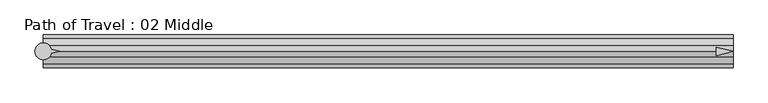
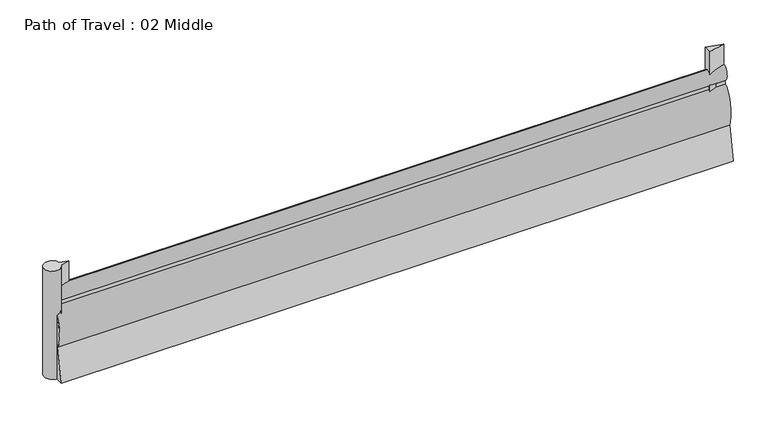
"""IFC4 building model written with IfcOpenShell, lengths in millimetres: proxy geometry, Path of Travel : 02 Middle."""

from ifc_helpers import new_model, si_unit, point, frame, frame_2d, origin, origin_with_axes, place, context, project, spatial, polyline, circle_curve, ellipse_curve, trimmed, segment, composite_curve, outline, extrude, source, transform, mapped, element, save
from ifc_brep_helpers import plane_surface, extruded_surface, advanced_brep


def path_of_travel_02_middle_b8d1a797(model_context):
    return source(origin(), model_context, "Body", "SolidModel", [
        advanced_brep(
        [(227.5554837, 0.0, 1727.2), (227.5554837, 42.9018657, 1436.6534209), (227.5554837, 42.9018657, 1363.4763406), (227.5554837, 184.1186263, 643.4144547), (227.5554837, 297.5699544, 0.0), (227.5554837, 145.6574193, 0.0), (227.5554837, 0.0, 584.2), (227.5554837, -145.6574193, 0.0), (227.5554837, -297.5699544, 0.0), (227.5554837, -184.1186263, 643.4144547), (227.5554837, -42.9018657, 1363.4763406), (227.5554837, -42.9018657, 1436.6534209), (12742.5650369, 0.0, 1727.2), (12742.5650369, -42.9018657, 1436.6534209), (12742.5650369, -42.9018657, 1363.4763406), (12742.5650369, -184.1186263, 643.4144547), (12742.5650369, -297.5699544, 0.0), (12742.5650369, -145.6574193, 0.0), (12742.5650369, 0.0, 584.2), (12742.5650369, 145.6574193, 0.0), (12742.5650369, 297.5699544, 0.0), (12742.5650369, 184.1186263, 643.4144547), (12742.5650369, 42.9018657, 1363.4763406), (12742.5650369, 42.9018657, 1436.6534209)],
        [
            (0, 1, ellipse_curve(frame((227.5554837, 0.0, 1574.8), z_axis=(-1.0, 0.0, 0.0), x_axis=(0.0, 0.0, 1.0)), 152.4, 101.6)),
            (1, 2),
            (2, 3, ellipse_curve(frame((227.5554837, 0.0, 914.4), z_axis=(-1.0, 0.0, 0.0), x_axis=(0.0, 0.0, -1.0)), 457.2, 228.6)),
            (3, 4),
            (4, 5),
            (5, 6),
            (6, 7),
            (7, 8),
            (8, 9),
            (9, 10, ellipse_curve(frame((227.5554837, 0.0, 914.4), z_axis=(-1.0, 0.0, 0.0), x_axis=(0.0, 0.0, -1.0)), 457.2, 228.6)),
            (10, 11),
            (11, 0, ellipse_curve(frame((227.5554837, 0.0, 1574.8), z_axis=(-1.0, 0.0, 0.0), x_axis=(0.0, 0.0, 1.0)), 152.4, 101.6)),
            (12, 13, ellipse_curve(frame((12742.5650369, 0.0, 1574.8), z_axis=(1.0, 0.0, 0.0), x_axis=(0.0, 0.0, 1.0)), 152.4, 101.6)),
            (13, 14),
            (14, 15, ellipse_curve(frame((12742.5650369, 0.0, 914.4), z_axis=(1.0, 0.0, 0.0), x_axis=(0.0, 0.0, -1.0)), 457.2, 228.6)),
            (15, 16),
            (16, 17),
            (17, 18),
            (18, 19),
            (19, 20),
            (20, 21),
            (21, 22, ellipse_curve(frame((12742.5650369, 0.0, 914.4), z_axis=(1.0, 0.0, 0.0), x_axis=(0.0, 0.0, -1.0)), 457.2, 228.6)),
            (22, 23),
            (23, 12, ellipse_curve(frame((12742.5650369, 0.0, 1574.8), z_axis=(1.0, 0.0, 0.0), x_axis=(0.0, 0.0, 1.0)), 152.4, 101.6)),
            (0, 12),
            (23, 1),
            (22, 2),
            (21, 3),
            (20, 4),
            (19, 5),
            (18, 6),
            (17, 7),
            (16, 8),
            (15, 9),
            (14, 10),
            (13, 11),
        ],
        [
            plane_surface(frame((227.5554837, 0.0, 0.0), z_axis=(-1.0, 0.0, 0.0), x_axis=(0.0, 0.0, 1.0))),
            plane_surface(frame((12742.5650369, 0.0, 0.0), z_axis=(1.0, 0.0, 0.0), x_axis=(0.0, 0.0, 1.0))),
            extruded_surface(trimmed(ellipse_curve(frame((12742.5650369, 0.0, 1574.8), z_axis=(-1.0, 0.0, 0.0), x_axis=(0.0, 0.0, 1.0)), 152.4, 101.6), [point((12742.5650369, 0.0, 1727.2))], [point((12742.5650369, 42.9018657, 1436.6534209))], True, "CARTESIAN"), (-12515.0095532, 0.0, 0.0), 12515.0095532),
            plane_surface(frame((227.5554837, 42.9018657, 1436.6534209), z_axis=(0.0, 1.0, 0.0), x_axis=(1.0, 0.0, 0.0))),
            extruded_surface(trimmed(ellipse_curve(frame((12742.5650369, 0.0, 914.4), z_axis=(-1.0, 0.0, 0.0), x_axis=(0.0, 0.0, -1.0)), 457.2, 228.6), [point((12742.5650369, 42.9018657, 1363.4763406))], [point((12742.5650369, 184.1186263, 643.4144547))], True, "CARTESIAN"), (-12515.0095532, 0.0, 0.0), 12515.0095532),
            plane_surface(frame((227.5554837, 184.1186263, 643.4144547), z_axis=(0.0, 0.9848077530122078, 0.1736481776669322), x_axis=(1.0, 0.0, 0.0))),
            plane_surface(frame((227.5554837, 297.5699544, 0.0), z_axis=(0.0, 0.0, -1.0), x_axis=(1.0, 0.0, 0.0))),
            plane_surface(frame((227.5554837, 145.6574193, 0.0), z_axis=(0.0, -0.9702957262760199, -0.2419218955995739), x_axis=(1.0, 0.0, 0.0))),
            plane_surface(frame((227.5554837, 0.0, 584.2), z_axis=(0.0, 0.9702957262759961, -0.24192189559966923), x_axis=(1.0, 0.0, 0.0))),
            plane_surface(frame((227.5554837, -145.6574193, 0.0), z_axis=(0.0, 0.0, -1.0), x_axis=(1.0, 0.0, 0.0))),
            plane_surface(frame((227.5554837, -297.5699544, 0.0), z_axis=(0.0, -0.984807753012208, 0.17364817766693066), x_axis=(1.0, 0.0, 0.0))),
            extruded_surface(trimmed(ellipse_curve(frame((12742.5650369, 0.0, 914.4), z_axis=(-1.0, 0.0, 0.0), x_axis=(0.0, 0.0, -1.0)), 457.2, 228.6), [point((12742.5650369, -184.1186263, 643.4144547))], [point((12742.5650369, -42.9018657, 1363.4763406))], True, "CARTESIAN"), (-12515.0095532, 0.0, 0.0), 12515.0095532),
            plane_surface(frame((227.5554837, -42.9018657, 1363.4763406), z_axis=(0.0, -1.0, 0.0), x_axis=(1.0, 0.0, 0.0))),
            extruded_surface(trimmed(ellipse_curve(frame((12742.5650369, 0.0, 1574.8), z_axis=(-1.0, 0.0, 0.0), x_axis=(0.0, 0.0, 1.0)), 152.4, 101.6), [point((12742.5650369, -42.9018657, 1436.6534209))], [point((12742.5650369, 0.0, 1727.2))], True, "CARTESIAN"), (-12515.0095532, 0.0, 0.0), 12515.0095532),
        ],
        [
            (0, [[1, 2, 3, 4, 5, 6, 7, 8, 9, 10, 11, 12]]),
            (1, [[13, 14, 15, 16, 17, 18, 19, 20, 21, 22, 23, 24]]),
            (2, [[-1, 25, -24, 26]]),
            (3, [[-2, -26, -23, 27]]),
            (4, [[-3, -27, -22, 28]]),
            (5, [[-4, -28, -21, 29]]),
            (6, [[-5, -29, -20, 30]]),
            (7, [[-6, -30, -19, 31]]),
            (8, [[-7, -31, -18, 32]]),
            (9, [[-8, -32, -17, 33]]),
            (10, [[-9, -33, -16, 34]]),
            (11, [[-10, -34, -15, 35]]),
            (12, [[-11, -35, -14, 36]]),
            (13, [[-12, -36, -13, -25]]),
        ],
    ),
        extrude(outline(polyline([(12436.5598904, 76.2006338), (12742.5650369, 0.0), (12436.5598904, -76.2006338), (12436.5598904, 76.2006338)])), origin_with_axes(), (0.0, 0.0, 1.0), 2129.5973753),
        extrude(outline(composite_curve([segment(polyline([(372.7837828, 39.4440225), (531.182385, 0.0), (372.7837828, -39.4440225)]), True, "CONTINUOUS"), segment(trimmed(circle_curve(frame_2d((227.2200886, 0.0)), 150.8131956), [point((372.7837828, -39.4440225))], [point((372.7837828, 39.4440225))], False, "CARTESIAN"), True, "CONTINUOUS")], self_intersect=False)), origin_with_axes(), (0.0, 0.0, 1.0), 2129.5973753),
    ])


if __name__ == "__main__":
    model = new_model("IFC4")
    model_context = context("Model", 3, world=origin())
    ifc_project = project(units=[si_unit("LENGTHUNIT", "METRE", prefix="MILLI")], contexts=[model_context])
    site = spatial("IfcSite", under=ifc_project)
    building = spatial("IfcBuilding", under=site)
    placement = place(None, origin())
    path_of_travel_02_middle_shape = path_of_travel_02_middle_b8d1a797(model_context)
    element("IfcBuildingElementProxy", 1, Name="Path of Travel : 02 Middle", ObjectType="Path of Travel : 02 Middle", at=placement, inside=building, context=model_context, shape_type="MappedRepresentation", body=[
        mapped(path_of_travel_02_middle_shape, transform((0.0, 0.0, 0.0), x_axis=(1.0, 0.0, 0.0), y_axis=(0.0, 1.0, 0.0), z_axis=(0.0, 0.0, 1.0))),
    ])
    save(model, "model.ifc")

# Revit data of these elements
# Type "Path of Travel : 02 Middle"
#   Path of Egress [instance default] = 4' - 0"
#   built-in parameter 1001306 [instance default] = 4 (stored number, unit not read)
#   Dot at Start = no
#   Arrow in Middle = yes
#   Arrow at End = no
#   Egress Path = none
# Element 1 (IfcBuildingElementProxy, "Path of Travel : 02 Middle")
#   Path of Egress = 41' - 0.71691"
#   built-in parameter 1001306 = 41.0597 (stored number, unit not read)
